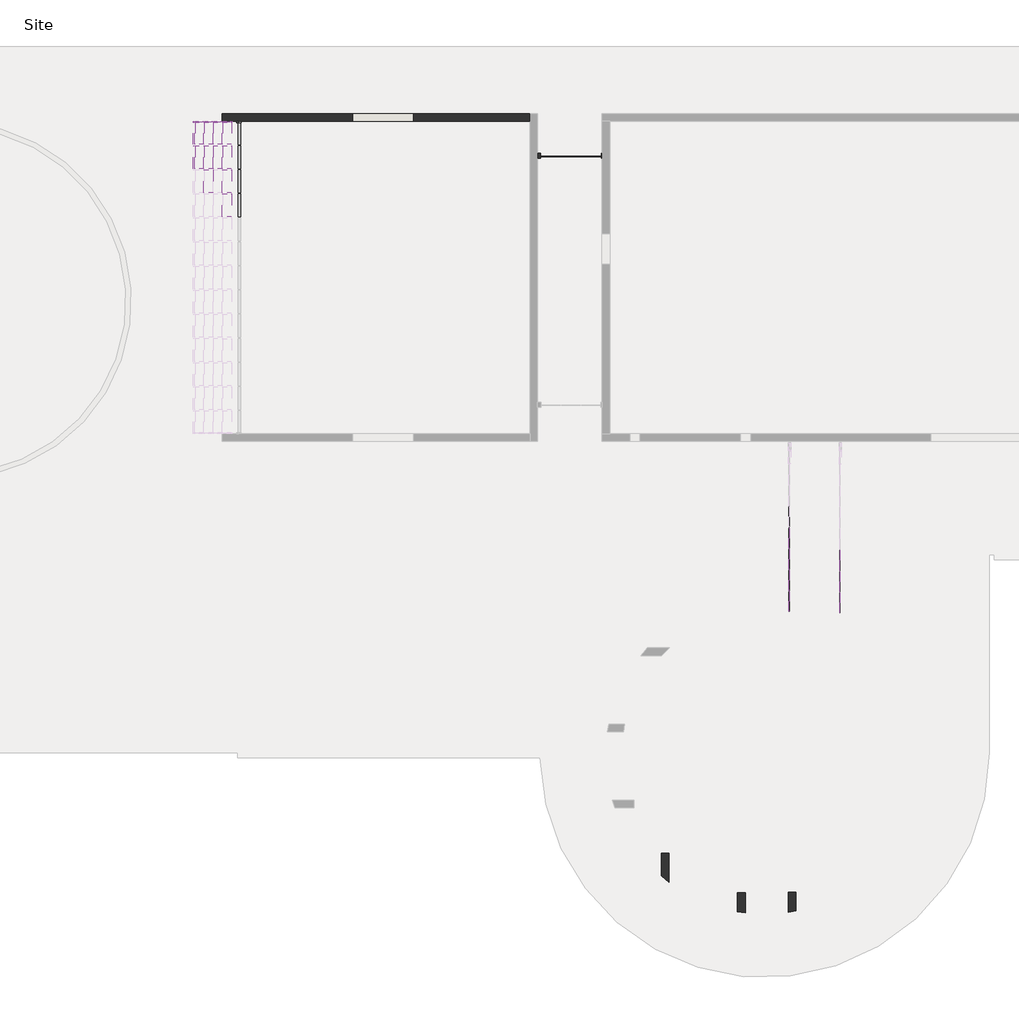
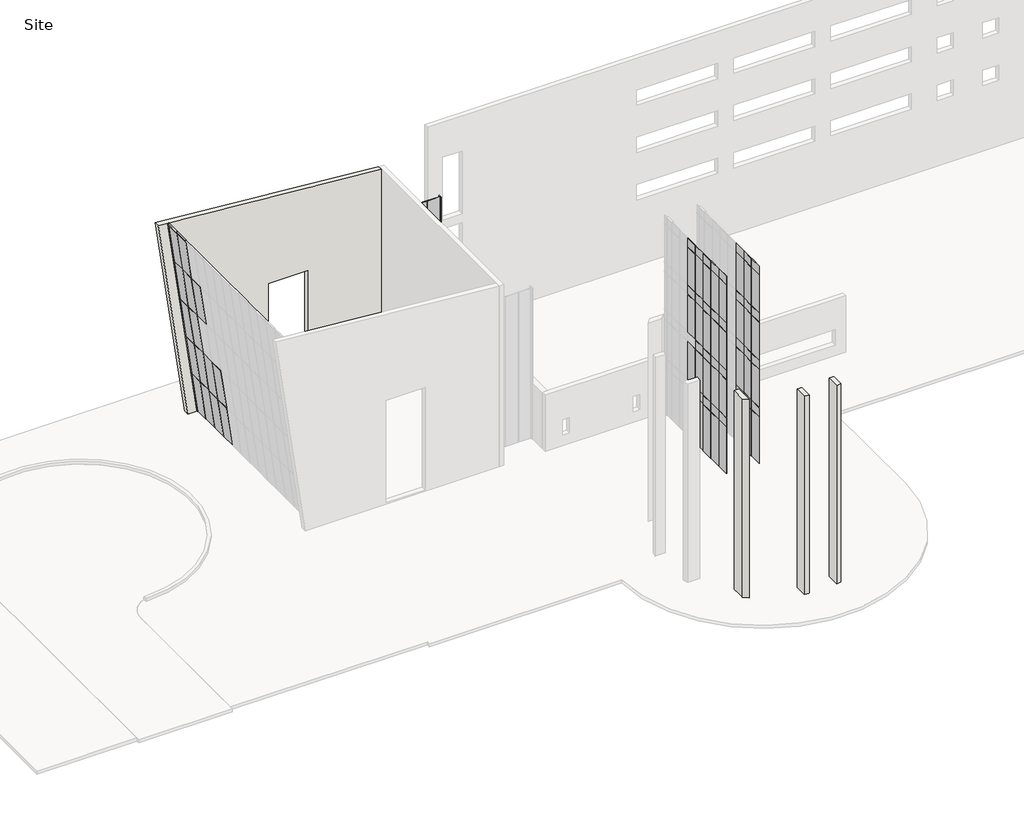
# One storey, part 2 of 4: 80 plates, 7 members, 6 walls.
"""IFC4 building model written with IfcOpenShell, lengths in millimetres."""

import ifcopenshell
import ifcopenshell.guid

model = None  # the IFC model being written
_history = None  # IfcOwnerHistory: only IFC2X3 demands one
_inside = {}  # id of a spatial element -> (the spatial element, [elements in it])
_under = {}  # id of a project, library or spatial element -> (it, [spatial elements below it])
_declared = {}  # id of a project -> (the project, [libraries it declares])
_typed = {}  # id of a type object -> (the type object, [elements of that type])
_made_of = {}  # id of a material, layer set ... -> (it, [elements and type objects made of it])


def new_model(schema):
    """Start an empty IFC model of exactly this schema.

    Asked for "IFC4X3", IfcOpenShell would pick the latest addendum, in which some entities
    have other attributes; the version numbers below select the first issue.
    IFC2X3 requires an IfcOwnerHistory on every rooted entity: one is made here for all.
    """
    global model, _history
    if schema == "IFC4X3":
        model = ifcopenshell.file(schema_version=(4, 3, 0, 0))
    else:
        model = ifcopenshell.file(schema=schema)
    _inside.clear()
    _under.clear()
    _declared.clear()
    _typed.clear()
    _made_of.clear()
    _history = None
    if model.schema == "IFC2X3":
        org = make("IfcOrganization", Name="unknown")
        user = make(
            "IfcPersonAndOrganization",
            ThePerson=make("IfcPerson", FamilyName="unknown"),
            TheOrganization=org,
        )
        app = make(
            "IfcApplication",
            ApplicationDeveloper=org,
            Version="unknown",
            ApplicationFullName="unknown",
            ApplicationIdentifier="unknown",
        )
        _history = make(
            "IfcOwnerHistory",
            OwningUser=user,
            OwningApplication=app,
            ChangeAction="ADDED",
            CreationDate=0,
        )
    return model


def make(cls, **values):
    """One entity of the class cls with the attributes given. An attribute that is None is left unset."""
    return model.create_entity(
        cls, **{name: value for name, value in values.items() if value is not None}
    )


def rooted(cls, **values):
    """An entity with a GlobalId (a new one), such as an element, a storey or a relation."""
    return make(cls, GlobalId=ifcopenshell.guid.new(), OwnerHistory=_history, **values)


def si_unit(unit_type, name, prefix=None):
    """IfcSIUnit, for example si_unit("LENGTHUNIT", "METRE", prefix="MILLI")."""
    return make("IfcSIUnit", UnitType=unit_type, Prefix=prefix, Name=name)


def assignment(units):
    """IfcUnitAssignment: the units of a project."""
    return None if units is None else make("IfcUnitAssignment", Units=units)


def point(xyz):
    """IfcCartesianPoint."""
    return None if xyz is None else make("IfcCartesianPoint", Coordinates=xyz)


def direction(xyz):
    """IfcDirection."""
    return None if xyz is None else make("IfcDirection", DirectionRatios=xyz)


def frame(location, z_axis=None, x_axis=None):
    """IfcAxis2Placement3D, a coordinate frame: its origin and axes. An axis left out is left unset."""
    return make(
        "IfcAxis2Placement3D",
        Location=point(location),
        Axis=direction(z_axis),
        RefDirection=direction(x_axis),
    )


def frame_2d(location, x_axis=None):
    """IfcAxis2Placement2D, a coordinate frame in the plane: its origin and x axis."""
    return make(
        "IfcAxis2Placement2D", Location=point(location), RefDirection=direction(x_axis)
    )


def origin():
    """The frame at (0, 0, 0) with its axes left unset."""
    return frame((0.0, 0.0, 0.0))


def origin_with_axes():
    """The frame at (0, 0, 0) with the z axis (0, 0, 1) and the x axis (1, 0, 0) written out."""
    return frame((0.0, 0.0, 0.0), z_axis=(0.0, 0.0, 1.0), x_axis=(1.0, 0.0, 0.0))


def place(relative_to, where):
    """IfcLocalPlacement: puts the frame where relative to a parent placement (None: the world)."""
    return make(
        "IfcLocalPlacement", PlacementRelTo=relative_to, RelativePlacement=where
    )


def context(
    kind, dimensions, precision=None, world=None, true_north=None, identifier=None
):
    """IfcGeometricRepresentationContext, for example the 3D "Model" context."""
    return make(
        "IfcGeometricRepresentationContext",
        ContextIdentifier=identifier,
        ContextType=kind,
        CoordinateSpaceDimension=dimensions,
        Precision=precision,
        WorldCoordinateSystem=world,
        TrueNorth=true_north,
    )


def project(units=None, contexts=None):
    """IfcProject with its units and contexts."""
    return rooted(
        "IfcProject",
        Name="project",
        RepresentationContexts=contexts,
        UnitsInContext=assignment(units),
    )


def spatial(cls, under=None, at=None, **own):
    """A site, building, storey or space (cls), placed at a placement, below another one or the project."""
    s = rooted(cls, ObjectPlacement=at, **own)
    if under is not None:
        _under.setdefault(under.id(), (under, []))[1].append(s)
    return s


def polyline(points):
    """IfcPolyline through the points."""
    return make("IfcPolyline", Points=[point(p) for p in points])


def circle_curve(where, radius):
    """IfcCircle in the frame where."""
    return make("IfcCircle", Position=where, Radius=radius)


def trimmed(basis, trim1, trim2, sense, master):
    """IfcTrimmedCurve: the piece of a basis curve between two trims."""
    return make(
        "IfcTrimmedCurve",
        BasisCurve=basis,
        Trim1=trim1,
        Trim2=trim2,
        SenseAgreement=sense,
        MasterRepresentation=master,
    )


def segment(curve, same_sense, transition):
    """IfcCompositeCurveSegment."""
    return make(
        "IfcCompositeCurveSegment",
        Transition=transition,
        SameSense=same_sense,
        ParentCurve=curve,
    )


def composite_curve(segments, self_intersect=None):
    """IfcCompositeCurve: segments joined end to end."""
    return make("IfcCompositeCurve", Segments=segments, SelfIntersect=self_intersect)


def outline(outer, holes=None, kind="AREA"):
    """IfcArbitraryClosedProfileDef: a profile drawn as a closed curve; with holes, ...WithVoids."""
    if holes is None:
        return make("IfcArbitraryClosedProfileDef", ProfileType=kind, OuterCurve=outer)
    return make(
        "IfcArbitraryProfileDefWithVoids",
        ProfileType=kind,
        OuterCurve=outer,
        InnerCurves=holes,
    )


def extrude(swept, where, along, depth):
    """IfcExtrudedAreaSolid: the profile swept, set in the frame where, extruded along a direction by depth."""
    return make(
        "IfcExtrudedAreaSolid",
        SweptArea=swept,
        Position=where,
        ExtrudedDirection=direction(along),
        Depth=depth,
    )


def shape(context_of_items, identifier, shape_type, items):
    """IfcShapeRepresentation: the items that make up one representation, for example the "Body"."""
    return make(
        "IfcShapeRepresentation",
        ContextOfItems=context_of_items,
        RepresentationIdentifier=identifier,
        RepresentationType=shape_type,
        Items=items,
    )


def source(mapping_origin, context_of_items, identifier, shape_type, items):
    """IfcRepresentationMap: a shape defined once, which mapped items show again and again."""
    return make(
        "IfcRepresentationMap",
        MappingOrigin=mapping_origin,
        MappedRepresentation=shape(context_of_items, identifier, shape_type, items),
    )


def transform(
    local_origin,
    x_axis=None,
    y_axis=None,
    z_axis=None,
    scale=None,
    scale2=None,
    scale3=None,
    uniform=True,
):
    """IfcCartesianTransformationOperator3D, or its non-uniform kind. x_axis, y_axis, z_axis: its Axis1, 2, 3."""
    if uniform:
        return make(
            "IfcCartesianTransformationOperator3D",
            Axis1=direction(x_axis),
            Axis2=direction(y_axis),
            LocalOrigin=point(local_origin),
            Scale=scale,
            Axis3=direction(z_axis),
        )
    return make(
        "IfcCartesianTransformationOperator3DnonUniform",
        Axis1=direction(x_axis),
        Axis2=direction(y_axis),
        LocalOrigin=point(local_origin),
        Scale=scale,
        Axis3=direction(z_axis),
        Scale2=scale2,
        Scale3=scale3,
    )


def mapped(mapping_source, mapping_target):
    """IfcMappedItem: shows the shape of a source again, moved by a transform."""
    return make(
        "IfcMappedItem", MappingSource=mapping_source, MappingTarget=mapping_target
    )


def made_of(thing, what):
    """Note that an element or type object is made of a material, layer set ...; save() writes the relation."""
    if what is not None:
        _made_of.setdefault(what.id(), (what, []))[1].append(thing)
    return thing


def element(
    cls,
    number,
    at=None,
    inside=None,
    cuts=None,
    type_object=None,
    material=None,
    context=None,
    identifier="Body",
    shape_type=None,
    held_by="IfcProductDefinitionShape",
    body=None,
    shapes=None,
    **own,
):
    """One element of the class cls, such as IfcWall. Its Tag is "e" and its number.

    at: its placement. inside: the storey or other place that contains it. cuts: it is an
    opening in that element (IfcRelVoidsElement). A single representation is given by context,
    identifier, shape_type and body (its items); several are given by shapes. held_by: the class
    of the entity that holds the representations. save() writes the other relations.
    """
    e = rooted(cls, Tag="e%d" % number, ObjectPlacement=at, **own)
    if body is not None:
        shapes = [shape(context, identifier, shape_type, body)]
    if shapes is not None:
        e.Representation = make(held_by, Representations=shapes)
    if inside is not None:
        _inside.setdefault(inside.id(), (inside, []))[1].append(e)
    if cuts is not None:
        rooted(
            "IfcRelVoidsElement", RelatingBuildingElement=cuts, RelatedOpeningElement=e
        )
    if type_object is not None:
        _typed.setdefault(type_object.id(), (type_object, []))[1].append(e)
    return made_of(e, material)


def aggregate(whole, parts):
    """IfcRelAggregates: a whole, such as a stair, and the parts it consists of."""
    return rooted("IfcRelAggregates", RelatingObject=whole, RelatedObjects=parts)


def save(model, path):
    """Write the relations noted so far, then the file.

    IfcRelAggregates (storeys below a building ...), IfcRelContainedInSpatialStructure (elements
    in a storey), IfcRelDefinesByType, IfcRelAssociatesMaterial and IfcRelDeclares: one each for
    every whole, place, type object, material and project.
    """
    for whole, parts in _under.values():
        aggregate(whole, parts)
    for where, things in _inside.values():
        rooted(
            "IfcRelContainedInSpatialStructure",
            RelatedElements=things,
            RelatingStructure=where,
        )
    for kind, things in _typed.values():
        rooted("IfcRelDefinesByType", RelatedObjects=things, RelatingType=kind)
    for what, things in _made_of.values():
        rooted("IfcRelAssociatesMaterial", RelatedObjects=things, RelatingMaterial=what)
    for by, libraries in _declared.values():
        rooted("IfcRelDeclares", RelatingContext=by, RelatedDefinitions=libraries)
    model.write(path)


def member_f8a9089e(model_context):
    return source(origin(), model_context, "Body", "SweptSolid", [
        extrude(outline(polyline([(0.0, 63.5), (0.0, -63.5), (-63.5, -63.5), (-63.5, 63.5), (0.0, 63.5)])), frame((0.0, 0.0, -1320.067308), z_axis=(0.0, 0.0, 1.0), x_axis=(1.0, 0.0, 0.0)), (0.0, 0.0, 1.0), 1320.067308),
    ])


def member_5e02c13a(model_context):
    return source(origin(), model_context, "Body", "SweptSolid", [
        extrude(outline(polyline([(0.0, 63.5), (0.0, -63.5), (-63.5, -63.5), (-63.5, 63.5), (0.0, 63.5)])), frame((0.0, 0.0, -1383.5673076), z_axis=(0.0, 0.0, 1.0), x_axis=(1.0, 0.0, 0.0)), (0.0, 0.0, 1.0), 1383.5673076),
    ])


def member_50cd645d(model_context):
    return source(origin(), model_context, "Body", "SweptSolid", [
        extrude(outline(polyline([(0.0, 63.5), (0.0, -63.5), (-63.5, -63.5), (-63.5, 63.5), (0.0, 63.5)])), frame((0.0, 0.0, -4003.5335741), z_axis=(0.0, 0.0, 1.0), x_axis=(1.0, 0.0, 0.0)), (0.0, 0.0, 1.0), 4003.5335741),
    ])


def member_5d333a65(model_context):
    return source(origin(), model_context, "Body", "SweptSolid", [
        extrude(outline(polyline([(0.0, 63.5), (0.0, -63.5), (-63.5, -63.5), (-63.5, 63.5), (0.0, 63.5)])), frame((0.0, 0.0, -3971.7835741), z_axis=(0.0, 0.0, 1.0), x_axis=(1.0, 0.0, 0.0)), (0.0, 0.0, 1.0), 3971.7835741),
    ])


def system_panel_glazed_908aa4c7(model_context):
    return source(origin(), model_context, "Body", "SweptSolid", [
        extrude(outline(polyline([(593.725, 19.05), (-593.725, 19.05), (-593.725, 44.45), (593.725, 44.45), (593.725, 19.05)])), origin_with_axes(), (0.0, 0.0, 1.0), 4629.15),
    ])


def system_panel_glazed_38880ecf(model_context):
    return source(origin(), model_context, "Body", "SweptSolid", [
        extrude(outline(polyline([(587.8744819, 19.05), (-587.8744819, 19.05), (-587.8744819, 44.45), (587.8744819, 44.45), (587.8744819, 19.05)])), origin_with_axes(), (0.0, 0.0, 1.0), 4629.15),
    ])


def system_panel_glazed_26f8e022(model_context):
    return source(origin(), model_context, "Body", "SweptSolid", [
        extrude(outline(polyline([(603.7494819, 19.05), (-603.7494819, 19.05), (-603.7494819, 44.45), (603.7494819, 44.45), (603.7494819, 19.05)])), origin_with_axes(), (0.0, 0.0, 1.0), 4629.15),
    ])


def system_panel_glazed_31d10065(model_context):
    return source(origin(), model_context, "Body", "SweptSolid", [
        extrude(outline(polyline([(609.6, 19.05), (-609.6, 19.05), (-609.6, 44.45), (609.6, 44.45), (609.6, 19.05)])), origin_with_axes(), (0.0, 0.0, 1.0), 4629.15),
    ])


def system_panel_glazed_d00c2bb3(model_context):
    return source(origin(), model_context, "Body", "SweptSolid", [
        extrude(outline(polyline([(609.5367635, 19.05), (-609.5367635, 19.05), (-609.5367635, 44.45), (609.5367635, 44.45), (609.5367635, 19.05)])), origin_with_axes(), (0.0, 0.0, 1.0), 15087.6),
    ])


def system_panel_glazed_c11227ff(model_context):
    return source(origin(), model_context, "Body", "SweptSolid", [
        extrude(outline(polyline([(593.725, 19.05), (-593.725, 19.05), (-593.725, 44.45), (593.725, 44.45), (593.725, 19.05)])), origin_with_axes(), (0.0, 0.0, 1.0), 3746.5),
    ])


def system_panel_glazed_2b3d2baa(model_context):
    return source(origin(), model_context, "Body", "SweptSolid", [
        extrude(outline(polyline([(609.6, 19.05), (-609.6, 19.05), (-609.6, 44.45), (609.6, 44.45), (609.6, 19.05)])), origin_with_axes(), (0.0, 0.0, 1.0), 3746.5),
    ])


def system_panel_glazed_00a161e3(model_context):
    return source(origin(), model_context, "Body", "SweptSolid", [
        extrude(outline(polyline([(593.725, 19.05), (-593.725, 19.05), (-593.725, 44.45), (593.725, 44.45), (593.725, 19.05)])), origin_with_axes(), (0.0, 0.0, 1.0), 850.9),
    ])


def system_panel_glazed_8fe7ab7d(model_context):
    return source(origin(), model_context, "Body", "SweptSolid", [
        extrude(outline(polyline([(609.6, 19.05), (-609.6, 19.05), (-609.6, 44.45), (609.6, 44.45), (609.6, 19.05)])), origin_with_axes(), (0.0, 0.0, 1.0), 850.9),
    ])


def system_panel_glazed_2ccc015e(model_context):
    return source(origin(), model_context, "Body", "SweptSolid", [
        extrude(outline(polyline([(593.725, 19.05), (-593.725, 19.05), (-593.725, 44.45), (593.725, 44.45), (593.725, 19.05)])), origin_with_axes(), (0.0, 0.0, 1.0), 819.15),
    ])


def system_panel_glazed_636dec6d(model_context):
    return source(origin(), model_context, "Body", "SweptSolid", [
        extrude(outline(polyline([(609.6, 19.05), (-609.6, 19.05), (-609.6, 44.45), (609.6, 44.45), (609.6, 19.05)])), origin_with_axes(), (0.0, 0.0, 1.0), 819.15),
    ])


def system_panel_glazed_4a693619(model_context):
    return source(origin(), model_context, "Body", "SweptSolid", [
        extrude(outline(polyline([(587.8744819, 19.05), (-587.8744819, 19.05), (-587.8744819, 44.45), (587.8744819, 44.45), (587.8744819, 19.05)])), origin_with_axes(), (0.0, 0.0, 1.0), 3746.5),
    ])


def system_panel_glazed_35bb093a(model_context):
    return source(origin(), model_context, "Body", "SweptSolid", [
        extrude(outline(polyline([(603.7494819, 19.05), (-603.7494819, 19.05), (-603.7494819, 44.45), (603.7494819, 44.45), (603.7494819, 19.05)])), origin_with_axes(), (0.0, 0.0, 1.0), 3746.5),
    ])


def system_panel_glazed_f91df05e(model_context):
    return source(origin(), model_context, "Body", "SweptSolid", [
        extrude(outline(polyline([(660.033654, 19.05), (-660.033654, 19.05), (-660.033654, 44.45), (660.033654, 44.45), (660.033654, 19.05)])), origin_with_axes(), (0.0, 0.0, 1.0), 3908.2835741),
    ])


def system_panel_glazed_78b5b18d(model_context):
    return source(origin(), model_context, "Body", "SweptSolid", [
        extrude(outline(polyline([(691.7836538, 19.05), (-691.7836538, 19.05), (-691.7836538, 44.45), (691.7836538, 44.45), (691.7836538, 19.05)])), origin_with_axes(), (0.0, 0.0, 1.0), 3908.2835741),
    ])


def system_panel_metal_panel_ca084d4b(model_context):
    return source(origin(), model_context, "Body", "SweptSolid", [
        extrude(outline(polyline([(587.8744819, 19.05), (-587.8744819, 19.05), (-587.8744819, 44.45), (587.8744819, 44.45), (587.8744819, 19.05)])), origin_with_axes(), (0.0, 0.0, 1.0), 819.15),
    ])


def system_panel_metal_panel_947f48db(model_context):
    return source(origin(), model_context, "Body", "SweptSolid", [
        extrude(outline(polyline([(603.7494819, 19.05), (-603.7494819, 19.05), (-603.7494819, 44.45), (603.7494819, 44.45), (603.7494819, 19.05)])), origin_with_axes(), (0.0, 0.0, 1.0), 819.15),
    ])


def system_panel_metal_panel_f9c2a482(model_context):
    return source(origin(), model_context, "Body", "SweptSolid", [
        extrude(outline(polyline([(587.8744819, 19.05), (-587.8744819, 19.05), (-587.8744819, 44.45), (587.8744819, 44.45), (587.8744819, 19.05)])), origin_with_axes(), (0.0, 0.0, 1.0), 850.9),
    ])


def system_panel_metal_panel_dcd9a435(model_context):
    return source(origin(), model_context, "Body", "SweptSolid", [
        extrude(outline(polyline([(603.7494819, 19.05), (-603.7494819, 19.05), (-603.7494819, 44.45), (603.7494819, 44.45), (603.7494819, 19.05)])), origin_with_axes(), (0.0, 0.0, 1.0), 850.9),
    ])


model = new_model("IFC4")

# Units and contexts
model_context = context("Model", 3, world=origin())
ifc_project = project(units=[si_unit("LENGTHUNIT", "METRE", prefix="MILLI")], contexts=[model_context])

# Site, building, storey
site = spatial("IfcSite", under=ifc_project)
building = spatial("IfcBuilding", under=site)
storey = spatial("IfcBuildingStorey", under=building, Name="Site", Elevation=-152.4)

# Members
placement = place(None, origin())
member_shape = member_f8a9089e(model_context)
element("IfcMember", 1, ObjectType="Rectangular Mullion1 : 2.5\" x 5\" rectangular", at=placement, inside=storey, context=model_context, shape_type="MappedRepresentation", body=[
    mapped(member_shape, transform((-27908.8595656, 55983.1320811, 19574.3667708), x_axis=(-0.13917310096006533, 0.0, 0.9902680687415704), y_axis=(-0.9902680687415704, 0.0, -0.13917310096006533), z_axis=(0.0, -1.0, 0.0))),
])
member_2_shape = member_5e02c13a(model_context)
element("IfcMember", 2, ObjectType="Rectangular Mullion1 : 2.5\" x 5\" rectangular", at=placement, inside=storey, context=model_context, shape_type="MappedRepresentation", body=[
    mapped(member_2_shape, transform((-27908.8595656, 54536.0647734, 19574.3667708), x_axis=(-0.13917310096006533, 0.0, 0.9902680687415704), y_axis=(-0.9902680687415704, 0.0, -0.13917310096006533), z_axis=(0.0, -1.0, 0.0))),
])
member_3_shape = member_50cd645d(model_context)
element("IfcMember", 3, ObjectType="Rectangular Mullion1 : 2.5\" x 5\" rectangular", at=placement, inside=storey, context=model_context, shape_type="MappedRepresentation", body=[
    mapped(member_3_shape, transform((-27908.8595656, 57366.699389, 19574.3667708), x_axis=(0.0, 1.0, 0.0), y_axis=(-0.9902680687415703, 0.0, -0.13917310096006566), z_axis=(-0.13917310096006566, 0.0, 0.9902680687415703))),
])
element("IfcMember", 4, ObjectType="Rectangular Mullion1 : 2.5\" x 5\" rectangular", at=placement, inside=storey, context=model_context, shape_type="MappedRepresentation", body=[
    mapped(member_3_shape, transform((-25693.3790742, 57366.699389, 3810.4039622), x_axis=(0.0, 1.0, 0.0), y_axis=(-0.9902680687415704, 0.0, -0.13917310096006544), z_axis=(-0.1391731009600654, 0.0, 0.9902680687415703))),
])
member_4_shape = member_5d333a65(model_context)
element("IfcMember", 5, ObjectType="Rectangular Mullion1 : 2.5\" x 5\" rectangular", at=placement, inside=storey, context=model_context, shape_type="MappedRepresentation", body=[
    mapped(member_4_shape, transform((-26246.1445106, 57366.699389, 7743.5344115), x_axis=(0.0, 1.0, 0.0), y_axis=(-0.9902680687415703, 0.0, -0.13917310096006563), z_axis=(-0.1391731009600656, 0.0, 0.9902680687415701))),
])
element("IfcMember", 6, ObjectType="Rectangular Mullion1 : 2.5\" x 5\" rectangular", at=placement, inside=storey, context=model_context, shape_type="MappedRepresentation", body=[
    mapped(member_4_shape, transform((-26798.9099469, 57366.699389, 11676.6648609), x_axis=(0.0, 1.0, 0.0), y_axis=(-0.9902680687415704, 0.0, -0.13917310096006574), z_axis=(-0.13917310096006574, 0.0, 0.9902680687415704))),
])
element("IfcMember", 7, ObjectType="Rectangular Mullion1 : 2.5\" x 5\" rectangular", at=placement, inside=storey, context=model_context, shape_type="MappedRepresentation", body=[
    mapped(member_4_shape, transform((-27351.6753833, 57366.699389, 15609.7953102), x_axis=(0.0, 1.0, 0.0), y_axis=(-0.9902680687415705, 0.0, -0.13917310096006458), z_axis=(-0.13917310096006458, 0.0, 0.9902680687415705))),
])

# Plates
system_panel_glazed_shape = system_panel_glazed_908aa4c7(model_context)
element("IfcPlate", 8, ObjectType="System Panel : Glazed", at=placement, inside=storey, context=model_context, shape_type="MappedRepresentation", body=[
    mapped(system_panel_glazed_shape, transform((10878.8276119, 28482.136889, -88.9), x_axis=(0.0, 1.0, 0.0), y_axis=(-1.0, 0.0, 0.0), z_axis=(0.0, 0.0, 1.0))),
])
system_panel_glazed_2_shape = system_panel_glazed_38880ecf(model_context)
element("IfcPlate", 9, ObjectType="System Panel : Glazed", at=placement, inside=storey, context=model_context, shape_type="MappedRepresentation", body=[
    mapped(system_panel_glazed_2_shape, transform((7830.8276119, 28569.8946611, -88.9), x_axis=(0.0, 1.0, 0.0), y_axis=(-1.0, 0.0, 0.0), z_axis=(0.0, 0.0, 1.0))),
])
system_panel_glazed_3_shape = system_panel_glazed_26f8e022(model_context)
element("IfcPlate", 10, ObjectType="System Panel : Glazed", at=placement, inside=storey, context=model_context, shape_type="MappedRepresentation", body=[
    mapped(system_panel_glazed_3_shape, transform((7830.8276119, 33638.015516, -88.9), x_axis=(0.0, 1.0, 0.0), y_axis=(-1.0, 0.0, 0.0), z_axis=(0.0, 0.0, 1.0))),
])
element("IfcPlate", 11, ObjectType="System Panel : Glazed", at=placement, inside=storey, context=model_context, shape_type="MappedRepresentation", body=[
    mapped(system_panel_glazed_3_shape, transform((7830.8276119, 31096.0175885, -88.9), x_axis=(0.0, 1.0, 0.0), y_axis=(-1.0, 0.0, 0.0), z_axis=(0.0, 0.0, 1.0))),
])
element("IfcPlate", 12, ObjectType="System Panel : Glazed", at=placement, inside=storey, context=model_context, shape_type="MappedRepresentation", body=[
    mapped(system_panel_glazed_3_shape, transform((7830.8276119, 32367.0165522, -88.9), x_axis=(0.0, 1.0, 0.0), y_axis=(-1.0, 0.0, 0.0), z_axis=(0.0, 0.0, 1.0))),
])
element("IfcPlate", 13, ObjectType="System Panel : Glazed", at=placement, inside=storey, context=model_context, shape_type="MappedRepresentation", body=[
    mapped(system_panel_glazed_3_shape, transform((7830.8276119, 29825.0186248, -88.9), x_axis=(0.0, 1.0, 0.0), y_axis=(-1.0, 0.0, 0.0), z_axis=(0.0, 0.0, 1.0))),
])
system_panel_glazed_4_shape = system_panel_glazed_31d10065(model_context)
element("IfcPlate", 14, ObjectType="System Panel : Glazed", at=placement, inside=storey, context=model_context, shape_type="MappedRepresentation", body=[
    mapped(system_panel_glazed_4_shape, transform((10878.8276119, 31031.661889, -88.9), x_axis=(0.0, 1.0, 0.0), y_axis=(-1.0, 0.0, 0.0), z_axis=(0.0, 0.0, 1.0))),
])
element("IfcPlate", 15, ObjectType="System Panel : Glazed", at=placement, inside=storey, context=model_context, shape_type="MappedRepresentation", body=[
    mapped(system_panel_glazed_4_shape, transform((10878.8276119, 29748.961889, -88.9), x_axis=(0.0, 1.0, 0.0), y_axis=(-1.0, 0.0, 0.0), z_axis=(0.0, 0.0, 1.0))),
])
system_panel_glazed_5_shape = system_panel_glazed_d00c2bb3(model_context)
element("IfcPlate", 16, ObjectType="System Panel : Glazed", at=placement, inside=storey, context=model_context, shape_type="MappedRepresentation", body=[
    mapped(system_panel_glazed_5_shape, transform((-4081.74698, 55307.711889, -152.4), x_axis=(-1.0, 0.0, 0.0), y_axis=(0.0, -1.0, 0.0), z_axis=(0.0, 0.0, 1.0))),
])
element("IfcPlate", 17, ObjectType="System Panel : Glazed", at=placement, inside=storey, context=model_context, shape_type="MappedRepresentation", body=[
    mapped(system_panel_glazed_5_shape, transform((-6519.8940341, 55307.711889, -152.4), x_axis=(-1.0, 0.0, 0.0), y_axis=(0.0, -1.0, 0.0), z_axis=(0.0, 0.0, 1.0))),
])
element("IfcPlate", 18, ObjectType="System Panel : Glazed", at=placement, inside=storey, context=model_context, shape_type="MappedRepresentation", body=[
    mapped(system_panel_glazed_5_shape, transform((-5300.8205071, 55307.711889, -152.4), x_axis=(-1.0, 0.0, 0.0), y_axis=(0.0, -1.0, 0.0), z_axis=(0.0, 0.0, 1.0))),
])
system_panel_glazed_6_shape = system_panel_glazed_c11227ff(model_context)
element("IfcPlate", 19, ObjectType="System Panel : Glazed", at=placement, inside=storey, context=model_context, shape_type="MappedRepresentation", body=[
    mapped(system_panel_glazed_6_shape, transform((10878.8276119, 28482.136889, 14966.95), x_axis=(0.0, 1.0, 0.0), y_axis=(-1.0, 0.0, 0.0), z_axis=(0.0, 0.0, 1.0))),
])
element("IfcPlate", 20, ObjectType="System Panel : Glazed", at=placement, inside=storey, context=model_context, shape_type="MappedRepresentation", body=[
    mapped(system_panel_glazed_6_shape, transform((10878.8276119, 28482.136889, 10242.55), x_axis=(0.0, 1.0, 0.0), y_axis=(-1.0, 0.0, 0.0), z_axis=(0.0, 0.0, 1.0))),
])
element("IfcPlate", 21, ObjectType="System Panel : Glazed", at=placement, inside=storey, context=model_context, shape_type="MappedRepresentation", body=[
    mapped(system_panel_glazed_6_shape, transform((10878.8276119, 28482.136889, 5518.15), x_axis=(0.0, 1.0, 0.0), y_axis=(-1.0, 0.0, 0.0), z_axis=(0.0, 0.0, 1.0))),
])
system_panel_glazed_7_shape = system_panel_glazed_2b3d2baa(model_context)
element("IfcPlate", 22, ObjectType="System Panel : Glazed", at=placement, inside=storey, context=model_context, shape_type="MappedRepresentation", body=[
    mapped(system_panel_glazed_7_shape, transform((10878.8276119, 29748.961889, 14966.95), x_axis=(0.0, 1.0, 0.0), y_axis=(-1.0, 0.0, 0.0), z_axis=(0.0, 0.0, 1.0))),
])
element("IfcPlate", 23, ObjectType="System Panel : Glazed", at=placement, inside=storey, context=model_context, shape_type="MappedRepresentation", body=[
    mapped(system_panel_glazed_7_shape, transform((10878.8276119, 31031.661889, 14966.95), x_axis=(0.0, 1.0, 0.0), y_axis=(-1.0, 0.0, 0.0), z_axis=(0.0, 0.0, 1.0))),
])
element("IfcPlate", 24, ObjectType="System Panel : Glazed", at=placement, inside=storey, context=model_context, shape_type="MappedRepresentation", body=[
    mapped(system_panel_glazed_7_shape, transform((10878.8276119, 29748.961889, 10242.55), x_axis=(0.0, 1.0, 0.0), y_axis=(-1.0, 0.0, 0.0), z_axis=(0.0, 0.0, 1.0))),
])
element("IfcPlate", 25, ObjectType="System Panel : Glazed", at=placement, inside=storey, context=model_context, shape_type="MappedRepresentation", body=[
    mapped(system_panel_glazed_7_shape, transform((10878.8276119, 31031.661889, 10242.55), x_axis=(0.0, 1.0, 0.0), y_axis=(-1.0, 0.0, 0.0), z_axis=(0.0, 0.0, 1.0))),
])
element("IfcPlate", 26, ObjectType="System Panel : Glazed", at=placement, inside=storey, context=model_context, shape_type="MappedRepresentation", body=[
    mapped(system_panel_glazed_7_shape, transform((10878.8276119, 29748.961889, 5518.15), x_axis=(0.0, 1.0, 0.0), y_axis=(-1.0, 0.0, 0.0), z_axis=(0.0, 0.0, 1.0))),
])
element("IfcPlate", 27, ObjectType="System Panel : Glazed", at=placement, inside=storey, context=model_context, shape_type="MappedRepresentation", body=[
    mapped(system_panel_glazed_7_shape, transform((10878.8276119, 31031.661889, 5518.15), x_axis=(0.0, 1.0, 0.0), y_axis=(-1.0, 0.0, 0.0), z_axis=(0.0, 0.0, 1.0))),
])
system_panel_glazed_8_shape = system_panel_glazed_00a161e3(model_context)
element("IfcPlate", 28, ObjectType="System Panel : Glazed", at=placement, inside=storey, context=model_context, shape_type="MappedRepresentation", body=[
    mapped(system_panel_glazed_8_shape, transform((10878.8276119, 28482.136889, 9328.15), x_axis=(0.0, 1.0, 0.0), y_axis=(-1.0, 0.0, 0.0), z_axis=(0.0, 0.0, 1.0))),
])
element("IfcPlate", 29, ObjectType="System Panel : Glazed", at=placement, inside=storey, context=model_context, shape_type="MappedRepresentation", body=[
    mapped(system_panel_glazed_8_shape, transform((10878.8276119, 28482.136889, 4603.75), x_axis=(0.0, 1.0, 0.0), y_axis=(-1.0, 0.0, 0.0), z_axis=(0.0, 0.0, 1.0))),
])
element("IfcPlate", 30, ObjectType="System Panel : Glazed", at=placement, inside=storey, context=model_context, shape_type="MappedRepresentation", body=[
    mapped(system_panel_glazed_8_shape, transform((10878.8276119, 28482.136889, 14052.55), x_axis=(0.0, 1.0, 0.0), y_axis=(-1.0, 0.0, 0.0), z_axis=(0.0, 0.0, 1.0))),
])
system_panel_glazed_9_shape = system_panel_glazed_8fe7ab7d(model_context)
element("IfcPlate", 31, ObjectType="System Panel : Glazed", at=placement, inside=storey, context=model_context, shape_type="MappedRepresentation", body=[
    mapped(system_panel_glazed_9_shape, transform((10878.8276119, 29748.961889, 9328.15), x_axis=(0.0, 1.0, 0.0), y_axis=(-1.0, 0.0, 0.0), z_axis=(0.0, 0.0, 1.0))),
])
element("IfcPlate", 32, ObjectType="System Panel : Glazed", at=placement, inside=storey, context=model_context, shape_type="MappedRepresentation", body=[
    mapped(system_panel_glazed_9_shape, transform((10878.8276119, 31031.661889, 9328.15), x_axis=(0.0, 1.0, 0.0), y_axis=(-1.0, 0.0, 0.0), z_axis=(0.0, 0.0, 1.0))),
])
element("IfcPlate", 33, ObjectType="System Panel : Glazed", at=placement, inside=storey, context=model_context, shape_type="MappedRepresentation", body=[
    mapped(system_panel_glazed_9_shape, transform((10878.8276119, 29748.961889, 4603.75), x_axis=(0.0, 1.0, 0.0), y_axis=(-1.0, 0.0, 0.0), z_axis=(0.0, 0.0, 1.0))),
])
element("IfcPlate", 34, ObjectType="System Panel : Glazed", at=placement, inside=storey, context=model_context, shape_type="MappedRepresentation", body=[
    mapped(system_panel_glazed_9_shape, transform((10878.8276119, 31031.661889, 4603.75), x_axis=(0.0, 1.0, 0.0), y_axis=(-1.0, 0.0, 0.0), z_axis=(0.0, 0.0, 1.0))),
])
element("IfcPlate", 35, ObjectType="System Panel : Glazed", at=placement, inside=storey, context=model_context, shape_type="MappedRepresentation", body=[
    mapped(system_panel_glazed_9_shape, transform((10878.8276119, 29748.961889, 14052.55), x_axis=(0.0, 1.0, 0.0), y_axis=(-1.0, 0.0, 0.0), z_axis=(0.0, 0.0, 1.0))),
])
element("IfcPlate", 36, ObjectType="System Panel : Glazed", at=placement, inside=storey, context=model_context, shape_type="MappedRepresentation", body=[
    mapped(system_panel_glazed_9_shape, transform((10878.8276119, 31031.661889, 14052.55), x_axis=(0.0, 1.0, 0.0), y_axis=(-1.0, 0.0, 0.0), z_axis=(0.0, 0.0, 1.0))),
])
system_panel_glazed_10_shape = system_panel_glazed_2ccc015e(model_context)
element("IfcPlate", 37, ObjectType="System Panel : Glazed", at=placement, inside=storey, context=model_context, shape_type="MappedRepresentation", body=[
    mapped(system_panel_glazed_10_shape, transform((10878.8276119, 28482.136889, 18776.95), x_axis=(0.0, 1.0, 0.0), y_axis=(-1.0, 0.0, 0.0), z_axis=(0.0, 0.0, 1.0))),
])
system_panel_glazed_11_shape = system_panel_glazed_636dec6d(model_context)
element("IfcPlate", 38, ObjectType="System Panel : Glazed", at=placement, inside=storey, context=model_context, shape_type="MappedRepresentation", body=[
    mapped(system_panel_glazed_11_shape, transform((10878.8276119, 29748.961889, 18776.95), x_axis=(0.0, 1.0, 0.0), y_axis=(-1.0, 0.0, 0.0), z_axis=(0.0, 0.0, 1.0))),
])
element("IfcPlate", 39, ObjectType="System Panel : Glazed", at=placement, inside=storey, context=model_context, shape_type="MappedRepresentation", body=[
    mapped(system_panel_glazed_11_shape, transform((10878.8276119, 31031.661889, 18776.95), x_axis=(0.0, 1.0, 0.0), y_axis=(-1.0, 0.0, 0.0), z_axis=(0.0, 0.0, 1.0))),
])
system_panel_glazed_12_shape = system_panel_glazed_4a693619(model_context)
element("IfcPlate", 40, ObjectType="System Panel : Glazed", at=placement, inside=storey, context=model_context, shape_type="MappedRepresentation", body=[
    mapped(system_panel_glazed_12_shape, transform((7830.8276119, 28569.8946611, 5518.15), x_axis=(0.0, 1.0, 0.0), y_axis=(-1.0, 0.0, 0.0), z_axis=(0.0, 0.0, 1.0))),
])
element("IfcPlate", 41, ObjectType="System Panel : Glazed", at=placement, inside=storey, context=model_context, shape_type="MappedRepresentation", body=[
    mapped(system_panel_glazed_12_shape, transform((7830.8276119, 28569.8946611, 10242.55), x_axis=(0.0, 1.0, 0.0), y_axis=(-1.0, 0.0, 0.0), z_axis=(0.0, 0.0, 1.0))),
])
element("IfcPlate", 42, ObjectType="System Panel : Glazed", at=placement, inside=storey, context=model_context, shape_type="MappedRepresentation", body=[
    mapped(system_panel_glazed_12_shape, transform((7830.8276119, 28569.8946611, 14966.95), x_axis=(0.0, 1.0, 0.0), y_axis=(-1.0, 0.0, 0.0), z_axis=(0.0, 0.0, 1.0))),
])
system_panel_glazed_13_shape = system_panel_glazed_35bb093a(model_context)
element("IfcPlate", 43, ObjectType="System Panel : Glazed", at=placement, inside=storey, context=model_context, shape_type="MappedRepresentation", body=[
    mapped(system_panel_glazed_13_shape, transform((7830.8276119, 29825.0186248, 5518.15), x_axis=(0.0, 1.0, 0.0), y_axis=(-1.0, 0.0, 0.0), z_axis=(0.0, 0.0, 1.0))),
])
element("IfcPlate", 44, ObjectType="System Panel : Glazed", at=placement, inside=storey, context=model_context, shape_type="MappedRepresentation", body=[
    mapped(system_panel_glazed_13_shape, transform((7830.8276119, 31096.0175885, 5518.15), x_axis=(0.0, 1.0, 0.0), y_axis=(-1.0, 0.0, 0.0), z_axis=(0.0, 0.0, 1.0))),
])
element("IfcPlate", 45, ObjectType="System Panel : Glazed", at=placement, inside=storey, context=model_context, shape_type="MappedRepresentation", body=[
    mapped(system_panel_glazed_13_shape, transform((7830.8276119, 32367.0165522, 5518.15), x_axis=(0.0, 1.0, 0.0), y_axis=(-1.0, 0.0, 0.0), z_axis=(0.0, 0.0, 1.0))),
])
element("IfcPlate", 46, ObjectType="System Panel : Glazed", at=placement, inside=storey, context=model_context, shape_type="MappedRepresentation", body=[
    mapped(system_panel_glazed_13_shape, transform((7830.8276119, 33638.015516, 5518.15), x_axis=(0.0, 1.0, 0.0), y_axis=(-1.0, 0.0, 0.0), z_axis=(0.0, 0.0, 1.0))),
])
element("IfcPlate", 47, ObjectType="System Panel : Glazed", at=placement, inside=storey, context=model_context, shape_type="MappedRepresentation", body=[
    mapped(system_panel_glazed_13_shape, transform((7830.8276119, 29825.0186248, 10242.55), x_axis=(0.0, 1.0, 0.0), y_axis=(-1.0, 0.0, 0.0), z_axis=(0.0, 0.0, 1.0))),
])
element("IfcPlate", 48, ObjectType="System Panel : Glazed", at=placement, inside=storey, context=model_context, shape_type="MappedRepresentation", body=[
    mapped(system_panel_glazed_13_shape, transform((7830.8276119, 31096.0175885, 10242.55), x_axis=(0.0, 1.0, 0.0), y_axis=(-1.0, 0.0, 0.0), z_axis=(0.0, 0.0, 1.0))),
])
element("IfcPlate", 49, ObjectType="System Panel : Glazed", at=placement, inside=storey, context=model_context, shape_type="MappedRepresentation", body=[
    mapped(system_panel_glazed_13_shape, transform((7830.8276119, 32367.0165522, 10242.55), x_axis=(0.0, 1.0, 0.0), y_axis=(-1.0, 0.0, 0.0), z_axis=(0.0, 0.0, 1.0))),
])
element("IfcPlate", 50, ObjectType="System Panel : Glazed", at=placement, inside=storey, context=model_context, shape_type="MappedRepresentation", body=[
    mapped(system_panel_glazed_13_shape, transform((7830.8276119, 33638.015516, 10242.55), x_axis=(0.0, 1.0, 0.0), y_axis=(-1.0, 0.0, 0.0), z_axis=(0.0, 0.0, 1.0))),
])
element("IfcPlate", 51, ObjectType="System Panel : Glazed", at=placement, inside=storey, context=model_context, shape_type="MappedRepresentation", body=[
    mapped(system_panel_glazed_13_shape, transform((7830.8276119, 29825.0186248, 14966.95), x_axis=(0.0, 1.0, 0.0), y_axis=(-1.0, 0.0, 0.0), z_axis=(0.0, 0.0, 1.0))),
])
element("IfcPlate", 52, ObjectType="System Panel : Glazed", at=placement, inside=storey, context=model_context, shape_type="MappedRepresentation", body=[
    mapped(system_panel_glazed_13_shape, transform((7830.8276119, 31096.0175885, 14966.95), x_axis=(0.0, 1.0, 0.0), y_axis=(-1.0, 0.0, 0.0), z_axis=(0.0, 0.0, 1.0))),
])
element("IfcPlate", 53, ObjectType="System Panel : Glazed", at=placement, inside=storey, context=model_context, shape_type="MappedRepresentation", body=[
    mapped(system_panel_glazed_13_shape, transform((7830.8276119, 32367.0165522, 14966.95), x_axis=(0.0, 1.0, 0.0), y_axis=(-1.0, 0.0, 0.0), z_axis=(0.0, 0.0, 1.0))),
])
element("IfcPlate", 54, ObjectType="System Panel : Glazed", at=placement, inside=storey, context=model_context, shape_type="MappedRepresentation", body=[
    mapped(system_panel_glazed_13_shape, transform((7830.8276119, 33638.015516, 14966.95), x_axis=(0.0, 1.0, 0.0), y_axis=(-1.0, 0.0, 0.0), z_axis=(0.0, 0.0, 1.0))),
])
system_panel_glazed_14_shape = system_panel_glazed_f91df05e(model_context)
element("IfcPlate", 55, ObjectType="System Panel : Glazed", at=placement, inside=storey, context=model_context, shape_type="MappedRepresentation", body=[
    mapped(system_panel_glazed_14_shape, transform((-25145.0323838, 56643.165735, -91.285476), x_axis=(0.0, -1.0, 0.0), y_axis=(0.9902680687415704, 0.0, 0.13917310096006547), z_axis=(-0.13917310096006547, 0.0, 0.9902680687415704))),
])
element("IfcPlate", 56, ObjectType="System Panel : Glazed", at=placement, inside=storey, context=model_context, shape_type="MappedRepresentation", body=[
    mapped(system_panel_glazed_14_shape, transform((-25697.7978202, 56643.165735, 3841.8449733), x_axis=(0.0, -1.0, 0.0), y_axis=(0.9902680687415704, 0.0, 0.13917310096006533), z_axis=(-0.13917310096006533, 0.0, 0.9902680687415704))),
])
element("IfcPlate", 57, ObjectType="System Panel : Glazed", at=placement, inside=storey, context=model_context, shape_type="MappedRepresentation", body=[
    mapped(system_panel_glazed_14_shape, transform((-26250.5632565, 56643.165735, 7774.9754227), x_axis=(0.0, -1.0, 0.0), y_axis=(0.9902680687415704, 0.0, 0.13917310096006533), z_axis=(-0.13917310096006533, 0.0, 0.9902680687415704))),
])
element("IfcPlate", 58, ObjectType="System Panel : Glazed", at=placement, inside=storey, context=model_context, shape_type="MappedRepresentation", body=[
    mapped(system_panel_glazed_14_shape, transform((-26803.3286929, 56643.165735, 11708.105872), x_axis=(0.0, -1.0, 0.0), y_axis=(0.9902680687415704, 0.0, 0.13917310096006533), z_axis=(-0.13917310096006533, 0.0, 0.9902680687415704))),
])
element("IfcPlate", 59, ObjectType="System Panel : Glazed", at=placement, inside=storey, context=model_context, shape_type="MappedRepresentation", body=[
    mapped(system_panel_glazed_14_shape, transform((-27356.0941292, 56643.165735, 15641.2363214), x_axis=(0.0, -1.0, 0.0), y_axis=(0.9902680687415704, 0.0, 0.13917310096006533), z_axis=(-0.13917310096006533, 0.0, 0.9902680687415704))),
])
system_panel_glazed_15_shape = system_panel_glazed_78b5b18d(model_context)
element("IfcPlate", 60, ObjectType="System Panel : Glazed", at=placement, inside=storey, context=model_context, shape_type="MappedRepresentation", body=[
    mapped(system_panel_glazed_15_shape, transform((-25145.0323838, 55227.8484272, -91.285476), x_axis=(0.0, -1.0, 0.0), y_axis=(0.9902680687415704, 0.0, 0.13917310096006547), z_axis=(-0.13917310096006547, 0.0, 0.9902680687415704))),
])
element("IfcPlate", 61, ObjectType="System Panel : Glazed", at=placement, inside=storey, context=model_context, shape_type="MappedRepresentation", body=[
    mapped(system_panel_glazed_15_shape, transform((-25145.0323838, 53780.7811196, -91.285476), x_axis=(0.0, -1.0, 0.0), y_axis=(0.9902680687415704, 0.0, 0.13917310096006547), z_axis=(-0.13917310096006547, 0.0, 0.9902680687415704))),
])
element("IfcPlate", 62, ObjectType="System Panel : Glazed", at=placement, inside=storey, context=model_context, shape_type="MappedRepresentation", body=[
    mapped(system_panel_glazed_15_shape, transform((-25145.0323838, 52333.7138119, -91.285476), x_axis=(0.0, -1.0, 0.0), y_axis=(0.9902680687415704, 0.0, 0.13917310096006547), z_axis=(-0.13917310096006547, 0.0, 0.9902680687415704))),
])
element("IfcPlate", 63, ObjectType="System Panel : Glazed", at=placement, inside=storey, context=model_context, shape_type="MappedRepresentation", body=[
    mapped(system_panel_glazed_15_shape, transform((-25697.7978202, 55227.8484272, 3841.8449733), x_axis=(0.0, -1.0, 0.0), y_axis=(0.9902680687415704, 0.0, 0.13917310096006533), z_axis=(-0.13917310096006533, 0.0, 0.9902680687415704))),
])
element("IfcPlate", 64, ObjectType="System Panel : Glazed", at=placement, inside=storey, context=model_context, shape_type="MappedRepresentation", body=[
    mapped(system_panel_glazed_15_shape, transform((-25697.7978202, 53780.7811196, 3841.8449733), x_axis=(0.0, -1.0, 0.0), y_axis=(0.9902680687415704, 0.0, 0.13917310096006533), z_axis=(-0.13917310096006533, 0.0, 0.9902680687415704))),
])
element("IfcPlate", 65, ObjectType="System Panel : Glazed", at=placement, inside=storey, context=model_context, shape_type="MappedRepresentation", body=[
    mapped(system_panel_glazed_15_shape, transform((-25697.7978202, 52333.7138119, 3841.8449733), x_axis=(0.0, -1.0, 0.0), y_axis=(0.9902680687415704, 0.0, 0.13917310096006533), z_axis=(-0.13917310096006533, 0.0, 0.9902680687415704))),
])
element("IfcPlate", 66, ObjectType="System Panel : Glazed", at=placement, inside=storey, context=model_context, shape_type="MappedRepresentation", body=[
    mapped(system_panel_glazed_15_shape, transform((-26250.5632565, 55227.8484272, 7774.9754227), x_axis=(0.0, -1.0, 0.0), y_axis=(0.9902680687415704, 0.0, 0.13917310096006533), z_axis=(-0.13917310096006533, 0.0, 0.9902680687415704))),
])
element("IfcPlate", 67, ObjectType="System Panel : Glazed", at=placement, inside=storey, context=model_context, shape_type="MappedRepresentation", body=[
    mapped(system_panel_glazed_15_shape, transform((-26803.3286929, 55227.8484272, 11708.105872), x_axis=(0.0, -1.0, 0.0), y_axis=(0.9902680687415704, 0.0, 0.13917310096006533), z_axis=(-0.13917310096006533, 0.0, 0.9902680687415704))),
])
element("IfcPlate", 68, ObjectType="System Panel : Glazed", at=placement, inside=storey, context=model_context, shape_type="MappedRepresentation", body=[
    mapped(system_panel_glazed_15_shape, transform((-26803.3286929, 53780.7811196, 11708.105872), x_axis=(0.0, -1.0, 0.0), y_axis=(0.9902680687415704, 0.0, 0.13917310096006533), z_axis=(-0.13917310096006533, 0.0, 0.9902680687415704))),
])
element("IfcPlate", 69, ObjectType="System Panel : Glazed", at=placement, inside=storey, context=model_context, shape_type="MappedRepresentation", body=[
    mapped(system_panel_glazed_15_shape, transform((-27356.0941292, 55227.8484272, 15641.2363214), x_axis=(0.0, -1.0, 0.0), y_axis=(0.9902680687415704, 0.0, 0.13917310096006533), z_axis=(-0.13917310096006533, 0.0, 0.9902680687415704))),
])
system_panel_metal_panel_shape = system_panel_metal_panel_ca084d4b(model_context)
element("IfcPlate", 70, ObjectType="System Panel : Metal Panel", at=placement, inside=storey, context=model_context, shape_type="MappedRepresentation", body=[
    mapped(system_panel_metal_panel_shape, transform((7830.8276119, 28569.8946611, 18776.95), x_axis=(0.0, 1.0, 0.0), y_axis=(-1.0, 0.0, 0.0), z_axis=(0.0, 0.0, 1.0))),
])
system_panel_metal_panel_2_shape = system_panel_metal_panel_947f48db(model_context)
element("IfcPlate", 71, ObjectType="System Panel : Metal Panel", at=placement, inside=storey, context=model_context, shape_type="MappedRepresentation", body=[
    mapped(system_panel_metal_panel_2_shape, transform((7830.8276119, 29825.0186248, 18776.95), x_axis=(0.0, 1.0, 0.0), y_axis=(-1.0, 0.0, 0.0), z_axis=(0.0, 0.0, 1.0))),
])
element("IfcPlate", 72, ObjectType="System Panel : Metal Panel", at=placement, inside=storey, context=model_context, shape_type="MappedRepresentation", body=[
    mapped(system_panel_metal_panel_2_shape, transform((7830.8276119, 31096.0175885, 18776.95), x_axis=(0.0, 1.0, 0.0), y_axis=(-1.0, 0.0, 0.0), z_axis=(0.0, 0.0, 1.0))),
])
element("IfcPlate", 73, ObjectType="System Panel : Metal Panel", at=placement, inside=storey, context=model_context, shape_type="MappedRepresentation", body=[
    mapped(system_panel_metal_panel_2_shape, transform((7830.8276119, 32367.0165522, 18776.95), x_axis=(0.0, 1.0, 0.0), y_axis=(-1.0, 0.0, 0.0), z_axis=(0.0, 0.0, 1.0))),
])
element("IfcPlate", 74, ObjectType="System Panel : Metal Panel", at=placement, inside=storey, context=model_context, shape_type="MappedRepresentation", body=[
    mapped(system_panel_metal_panel_2_shape, transform((7830.8276119, 33638.015516, 18776.95), x_axis=(0.0, 1.0, 0.0), y_axis=(-1.0, 0.0, 0.0), z_axis=(0.0, 0.0, 1.0))),
])
system_panel_metal_panel_3_shape = system_panel_metal_panel_f9c2a482(model_context)
element("IfcPlate", 75, ObjectType="System Panel : Metal Panel", at=placement, inside=storey, context=model_context, shape_type="MappedRepresentation", body=[
    mapped(system_panel_metal_panel_3_shape, transform((7830.8276119, 28569.8946611, 14052.55), x_axis=(0.0, 1.0, 0.0), y_axis=(-1.0, 0.0, 0.0), z_axis=(0.0, 0.0, 1.0))),
])
element("IfcPlate", 76, ObjectType="System Panel : Metal Panel", at=placement, inside=storey, context=model_context, shape_type="MappedRepresentation", body=[
    mapped(system_panel_metal_panel_3_shape, transform((7830.8276119, 28569.8946611, 9328.15), x_axis=(0.0, 1.0, 0.0), y_axis=(-1.0, 0.0, 0.0), z_axis=(0.0, 0.0, 1.0))),
])
element("IfcPlate", 77, ObjectType="System Panel : Metal Panel", at=placement, inside=storey, context=model_context, shape_type="MappedRepresentation", body=[
    mapped(system_panel_metal_panel_3_shape, transform((7830.8276119, 28569.8946611, 4603.75), x_axis=(0.0, 1.0, 0.0), y_axis=(-1.0, 0.0, 0.0), z_axis=(0.0, 0.0, 1.0))),
])
system_panel_metal_panel_4_shape = system_panel_metal_panel_dcd9a435(model_context)
element("IfcPlate", 78, ObjectType="System Panel : Metal Panel", at=placement, inside=storey, context=model_context, shape_type="MappedRepresentation", body=[
    mapped(system_panel_metal_panel_4_shape, transform((7830.8276119, 29825.0186248, 14052.55), x_axis=(0.0, 1.0, 0.0), y_axis=(-1.0, 0.0, 0.0), z_axis=(0.0, 0.0, 1.0))),
])
element("IfcPlate", 79, ObjectType="System Panel : Metal Panel", at=placement, inside=storey, context=model_context, shape_type="MappedRepresentation", body=[
    mapped(system_panel_metal_panel_4_shape, transform((7830.8276119, 31096.0175885, 14052.55), x_axis=(0.0, 1.0, 0.0), y_axis=(-1.0, 0.0, 0.0), z_axis=(0.0, 0.0, 1.0))),
])
element("IfcPlate", 80, ObjectType="System Panel : Metal Panel", at=placement, inside=storey, context=model_context, shape_type="MappedRepresentation", body=[
    mapped(system_panel_metal_panel_4_shape, transform((7830.8276119, 32367.0165522, 14052.55), x_axis=(0.0, 1.0, 0.0), y_axis=(-1.0, 0.0, 0.0), z_axis=(0.0, 0.0, 1.0))),
])
element("IfcPlate", 81, ObjectType="System Panel : Metal Panel", at=placement, inside=storey, context=model_context, shape_type="MappedRepresentation", body=[
    mapped(system_panel_metal_panel_4_shape, transform((7830.8276119, 33638.015516, 14052.55), x_axis=(0.0, 1.0, 0.0), y_axis=(-1.0, 0.0, 0.0), z_axis=(0.0, 0.0, 1.0))),
])
element("IfcPlate", 82, ObjectType="System Panel : Metal Panel", at=placement, inside=storey, context=model_context, shape_type="MappedRepresentation", body=[
    mapped(system_panel_metal_panel_4_shape, transform((7830.8276119, 29825.0186248, 9328.15), x_axis=(0.0, 1.0, 0.0), y_axis=(-1.0, 0.0, 0.0), z_axis=(0.0, 0.0, 1.0))),
])
element("IfcPlate", 83, ObjectType="System Panel : Metal Panel", at=placement, inside=storey, context=model_context, shape_type="MappedRepresentation", body=[
    mapped(system_panel_metal_panel_4_shape, transform((7830.8276119, 31096.0175885, 9328.15), x_axis=(0.0, 1.0, 0.0), y_axis=(-1.0, 0.0, 0.0), z_axis=(0.0, 0.0, 1.0))),
])
element("IfcPlate", 84, ObjectType="System Panel : Metal Panel", at=placement, inside=storey, context=model_context, shape_type="MappedRepresentation", body=[
    mapped(system_panel_metal_panel_4_shape, transform((7830.8276119, 32367.0165522, 9328.15), x_axis=(0.0, 1.0, 0.0), y_axis=(-1.0, 0.0, 0.0), z_axis=(0.0, 0.0, 1.0))),
])
element("IfcPlate", 85, ObjectType="System Panel : Metal Panel", at=placement, inside=storey, context=model_context, shape_type="MappedRepresentation", body=[
    mapped(system_panel_metal_panel_4_shape, transform((7830.8276119, 29825.0186248, 4603.75), x_axis=(0.0, 1.0, 0.0), y_axis=(-1.0, 0.0, 0.0), z_axis=(0.0, 0.0, 1.0))),
])
element("IfcPlate", 86, ObjectType="System Panel : Metal Panel", at=placement, inside=storey, context=model_context, shape_type="MappedRepresentation", body=[
    mapped(system_panel_metal_panel_4_shape, transform((7830.8276119, 31096.0175885, 4603.75), x_axis=(0.0, 1.0, 0.0), y_axis=(-1.0, 0.0, 0.0), z_axis=(0.0, 0.0, 1.0))),
])
element("IfcPlate", 87, ObjectType="System Panel : Metal Panel", at=placement, inside=storey, context=model_context, shape_type="MappedRepresentation", body=[
    mapped(system_panel_metal_panel_4_shape, transform((7830.8276119, 32367.0165522, 4603.75), x_axis=(0.0, 1.0, 0.0), y_axis=(-1.0, 0.0, 0.0), z_axis=(0.0, 0.0, 1.0))),
])

# Walls
element("IfcWall", 88, ObjectType="Stone on CMU", at=placement, inside=storey, context=model_context, shape_type="SweptSolid", body=[
    extrude(outline(composite_curve([segment(polyline([(140.6953567, 12095.1176395), (140.6953567, 13452.4789718), (594.7203567, 13452.4789718), (594.7203567, 11730.5482318)]), True, "CONTINUOUS"), segment(trimmed(circle_curve(frame_2d((6332.5692024, 19341.311889)), 9531.35), [point((594.7203567, 11730.5482318))], [point((140.6953567, 12095.1176395))], False, "CARTESIAN"), True, "CONTINUOUS")], self_intersect=False)), frame((0.0, 0.0, -152.4), z_axis=(0.0, 0.0, 1.0), x_axis=(1.0, 0.0, 0.0)), (0.0, 0.0, 1.0), 19812.0),
])
element("IfcWall", 89, ObjectType="Stone on CMU", at=placement, inside=storey, context=model_context, shape_type="SweptSolid", body=[
    extrude(outline(composite_curve([segment(polyline([(4712.6953567, 9948.6210314), (4712.6953567, 11075.8499375), (5166.7203567, 11075.8499375), (5166.7203567, 9881.5323307)]), True, "CONTINUOUS"), segment(trimmed(circle_curve(frame_2d((6332.5692024, 19341.311889)), 9531.35), [point((5166.7203567, 9881.5323307))], [point((4712.6953567, 9948.6210314))], False, "CARTESIAN"), True, "CONTINUOUS")], self_intersect=False)), frame((0.0, 0.0, -152.4), z_axis=(0.0, 0.0, 1.0), x_axis=(1.0, 0.0, 0.0)), (0.0, 0.0, 1.0), 19812.0),
])
element("IfcWall", 90, ObjectType="Stone on CMU", at=placement, inside=storey, context=model_context, shape_type="SweptSolid", body=[
    extrude(outline(composite_curve([segment(polyline([(7760.6953567, 9917.5605919), (7760.6953567, 11124.3513783), (8214.7203567, 11124.3513783), (8214.7203567, 9997.6434523)]), True, "CONTINUOUS"), segment(trimmed(circle_curve(frame_2d((6332.5692024, 19341.311889)), 9531.35), [point((8214.7203567, 9997.6434523))], [point((7760.6953567, 9917.5605919))], False, "CARTESIAN"), True, "CONTINUOUS")], self_intersect=False)), frame((0.0, 0.0, -152.4), z_axis=(0.0, 0.0, 1.0), x_axis=(1.0, 0.0, 0.0)), (0.0, 0.0, 1.0), 19812.0),
])
element("IfcWall", 91, ObjectType="Stone on CMU", at=placement, inside=storey, context=model_context, shape_type="SweptSolid", body=[
    extrude(outline(polyline([(-152.4, -26050.8432976), (-152.4, -7761.2557976), (17898.2153222, -7761.2557976), (19654.3186785, -28834.4960734), (-152.4, -26050.8432976)]), holes=[polyline([(10210.8, -14747.8432976), (0.0, -14747.8432976), (0.0, -18405.4432976), (10210.8, -18405.4432976), (10210.8, -14747.8432976)])]), frame((0.0, 57366.699389, 0.0), z_axis=(0.0, 1.0, 0.0), x_axis=(0.0, 0.0, 1.0)), (0.0, 0.0, 1.0), 454.025),
])
element("IfcWall", 92, ObjectType="a_Mtl panel on Mtl stud", at=placement, inside=storey, context=model_context, shape_type="SweptSolid", body=[
    extrude(outline(polyline([(-3472.2102165, 55463.286889), (-3419.8227165, 55463.286889), (-3419.8227165, 55152.136889), (-3472.2102165, 55152.136889), (-3472.2102165, 55463.286889)])), frame((0.0, 0.0, -152.4), z_axis=(0.0, 0.0, 1.0), x_axis=(1.0, 0.0, 0.0)), (0.0, 0.0, 1.0), 15087.6),
])
element("IfcWall", 93, ObjectType="a_Mtl panel on Mtl stud", at=placement, inside=storey, context=model_context, shape_type="SweptSolid", body=[
    extrude(outline(polyline([(-7307.2307976, 55463.286889), (-7129.4307976, 55463.286889), (-7129.4307976, 55152.136889), (-7307.2307976, 55152.136889), (-7307.2307976, 55463.286889)])), frame((0.0, 0.0, -152.4), z_axis=(0.0, 0.0, 1.0), x_axis=(1.0, 0.0, 0.0)), (0.0, 0.0, 1.0), 15087.6),
])

save(model, "model.ifc")

# Revit data of these elements
# Project information
#   Project Issue Date = "Issue Date"
#   Project Status = "Project Status"
#   Client Name = "Owner"
#   Project Address = "Enter address here"
#   Project Name = "Project Name"
#   Project Number = "Project Number"
# Grids (mm)
#   "8": line (61272.769, 33542.122) -> (61272.769, 61407.715)
#   "7": line (52128.769, 33542.122) -> (52128.769, 61407.715)
#   "6": line (42984.769, 33542.122) -> (42984.769, 61407.715)
#   "5": line (33840.769, 33542.122) -> (33840.769, 61407.715)
#   "4": line (24696.769, 33542.122) -> (24696.769, 61407.715)
#   "3": line (15552.769, 33542.122) -> (15552.769, 61407.715)
#   "2": line (6408.769, 33542.122) -> (6408.769, 61407.715)
#   "1": line (-2735.231, 33542.122) -> (-2735.231, 61407.715)
#   "A": line (-6275.236, 57136.512) -> (64520.567, 57136.512)
#   "B": line (-6275.236, 47992.512) -> (64520.567, 47992.512)
#   "C": line (-6275.236, 38848.512) -> (64520.567, 38848.512)
# Type "Rectangular Mullion1 : 2.5\" x 5\" rectangular"
#   built-in parameter 1007304 = 0.416667 (stored number, unit not read)
#   built-in parameter 1007301 = 0.104167 (stored number, unit not read)
#   built-in parameter 1007300 = 0.104167 (stored number, unit not read)
# Type "System Panel : Glazed"
#   Construction Type Id = "GSP4R"
#   Analytic Construction = "1/8 in Pilkington single glazing"
#   Visual Light Transmittance = 0.9
#   Solar Heat Gain Coefficient = 0.86
#   Heat Transfer Coefficient (U) = 1.18115 BTU/(h·ft²·°F)
#   Define Thermal Properties by = 1
# Type "Stone on CMU"
#   Layers, outside or top first: 0' - 2" "Panel Granite 72x48" (function 4); 0' - 3" "Misc. Air Layers - Air Space" (function 3); 0' - 3" "Insulation / Thermal Barriers - Batt insulation" (function 3); 0' - 0" "Vapor / Moisture Barriers - Vapor Retarder" (function 100); 0' - 7 5/8" "Masonry - Concrete Masonry Units" (function 1); 0' - 1 5/8" "Metal - Furring" (function 2); 0' - 0 5/8" "Gypsum Wall Board" (function 5)
# Type "a_Mtl panel on Mtl stud"
#   Layers, outside or top first: 0' - 2" "Metal - Panel" (function 0); 0' - 3" "Misc. Air Layers - Air Space" (function 0); 0' - 0" "Air Barrier - Air Infiltration Barrier" (function 0); 0' - 0 3/4" "Wood - Sheathing - plywood" (function 0); 0' - 6" "Metal - Stud Layer" (function 0); 0' - 0" "Vapor / Moisture Barriers - Vapor Retarder" (function 0); 0' - 0 1/2" no material (function 0)
# Elements 1, 2, 3, 4, 5, 6, 7 (IfcMember, "Rectangular Mullion1 : 2.5\" x 5\" rectangular")
#   Phase Created = New Construction
#   Materials on its faces: "support-frame"
# Elements 8, 9, 10, 11, 12, 13, 14, 15, 16, 17, 18, 19, 20, 21, 22, 23, 24, 25, 26, 27, 28, 29, 30, 31, 32, 33, 34, 35, 36, 37, 38, 39, 40, 41, 42, 43, 44, 45, 46, 47, 48, 49, 50, 51, 52, 53, 54, 55, 56, 57, 58, 59, 60, 61, 62, 63, 64, 65, 66, 67, 68, 69 (IfcPlate, "System Panel : Glazed")
#   Phase Created = New Construction
#   Materials on its faces: "Glass"
# Elements 70, 71, 72, 73, 74, 75, 76, 77, 78, 79, 80, 81, 82, 83, 84, 85, 86, 87 (IfcPlate, "System Panel : Metal Panel")
#   Phase Created = New Construction
#   Materials on its faces: "Aluminum"
# Elements 88, 89, 90 (IfcWall, "Stone on CMU")
#   Top Offset = 0' - 0"
#   Base Offset = 0' - 0"
#   wall height = 65' - 0"
#   Phase Created = New Construction
#   Base Constraint = Site
#   Top Constraint = Roof
#   Materials on its faces: "Default Wall", "Gypsum Wall Board", "Panel Granite 72x48"
# Element 91 (IfcWall, "Stone on CMU")
#   Top Offset = 0' - 0"
#   Base Offset = 0' - 0"
#   wall height = 68' - 0"
#   Phase Created = New Construction
#   Base Constraint = Site
#   Top Constraint = Parapet
#   Materials on its faces: "Default Wall", "Panel Granite 72x48", "Gypsum Wall Board"
# Elements 92, 93 (IfcWall, "a_Mtl panel on Mtl stud")
#   Top Offset = 0' - 0"
#   Base Offset = 0' - 0"
#   wall height = 49' - 6"
#   Phase Created = New Construction
#   Base Constraint = Site
#   Top Constraint = Floor 4
#   Materials on its faces: "Default Wall", "Metal - Panel"
# Materials
#   "Panel Granite 72x48": class "Stone", colour RGB 226 230 231, transparency 0, Cost = 0
#   "Misc. Air Layers - Air Space": class "Miscellaneous", colour RGB 255 255 255, transparency 0
#   "Insulation / Thermal Barriers - Batt insulation": class "Unassigned", colour RGB 127 127 127, transparency 0, Comments = "Rendering appearance not upgraded ", Cost = 0
#   "Vapor / Moisture Barriers - Vapor Retarder": class "Miscellaneous", colour RGB 127 127 127, transparency 0
#   "Masonry - Concrete Masonry Units": class "Concrete", colour RGB 227 227 227, transparency 0
#   "Metal - Furring": class "Metal", colour RGB 199 199 199, transparency 0
#   "Gypsum Wall Board": class "Generic", colour RGB 127 127 127, transparency 0, Description = "Gypsum Wall Board", Cost = 0
#   "Metal - Panel": class "Unassigned", colour RGB 127 127 127, transparency 0
#   "Air Barrier - Air Infiltration Barrier": class "Miscellaneous", colour RGB 127 127 127, transparency 0
#   "Wood - Sheathing - plywood": class "Wood", colour RGB 212 179 113, transparency 0
#   "Metal - Stud Layer": class "Metal", colour RGB 199 199 199, transparency 0
#   "support-frame": class "Unassigned", colour RGB 233 233 233, transparency 0, Cost = 0
#   "Glass": class "Glass", colour RGB 0 128 192, transparency 0.75, Description = "Soda Lime Glass", Cost = 0
#   "Aluminum": class "Metal", colour RGB 247 247 247, transparency 0, Description = "Aluminum 6061", Cost = 0
#   "Default Wall": class "Miscellaneous", colour RGB 128 128 128, transparency 0, Cost = 0
